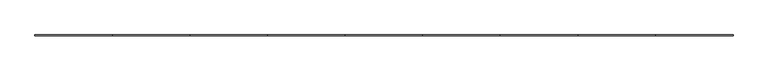
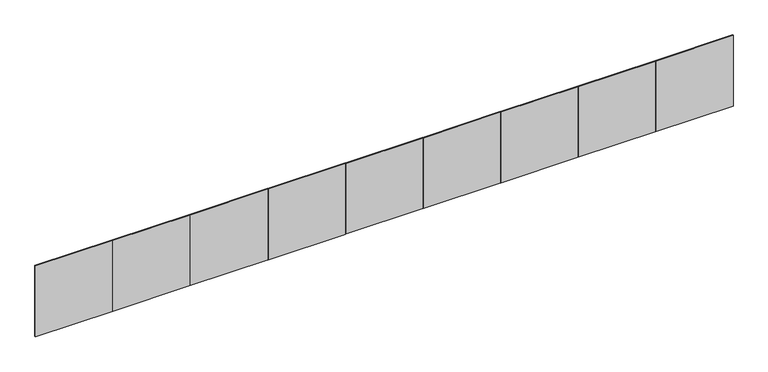
"""IFC4 building model written with IfcOpenShell, lengths in millimetres: railing geometry, ML_Painéis : ML_Painéis."""

import ifcopenshell
import ifcopenshell.guid

model = None  # the IFC model being written
_history = None  # IfcOwnerHistory: only IFC2X3 demands one
_inside = {}  # id of a spatial element -> (the spatial element, [elements in it])
_under = {}  # id of a project, library or spatial element -> (it, [spatial elements below it])
_declared = {}  # id of a project -> (the project, [libraries it declares])
_typed = {}  # id of a type object -> (the type object, [elements of that type])
_made_of = {}  # id of a material, layer set ... -> (it, [elements and type objects made of it])


def new_model(schema):
    """Start an empty IFC model of exactly this schema.

    Asked for "IFC4X3", IfcOpenShell would pick the latest addendum, in which some entities
    have other attributes; the version numbers below select the first issue.
    IFC2X3 requires an IfcOwnerHistory on every rooted entity: one is made here for all.
    """
    global model, _history
    if schema == "IFC4X3":
        model = ifcopenshell.file(schema_version=(4, 3, 0, 0))
    else:
        model = ifcopenshell.file(schema=schema)
    _inside.clear()
    _under.clear()
    _declared.clear()
    _typed.clear()
    _made_of.clear()
    _history = None
    if model.schema == "IFC2X3":
        org = make("IfcOrganization", Name="unknown")
        user = make(
            "IfcPersonAndOrganization",
            ThePerson=make("IfcPerson", FamilyName="unknown"),
            TheOrganization=org,
        )
        app = make(
            "IfcApplication",
            ApplicationDeveloper=org,
            Version="unknown",
            ApplicationFullName="unknown",
            ApplicationIdentifier="unknown",
        )
        _history = make(
            "IfcOwnerHistory",
            OwningUser=user,
            OwningApplication=app,
            ChangeAction="ADDED",
            CreationDate=0,
        )
    return model


def make(cls, **values):
    """One entity of the class cls with the attributes given. An attribute that is None is left unset."""
    return model.create_entity(
        cls, **{name: value for name, value in values.items() if value is not None}
    )


def rooted(cls, **values):
    """An entity with a GlobalId (a new one), such as an element, a storey or a relation."""
    return make(cls, GlobalId=ifcopenshell.guid.new(), OwnerHistory=_history, **values)


def si_unit(unit_type, name, prefix=None):
    """IfcSIUnit, for example si_unit("LENGTHUNIT", "METRE", prefix="MILLI")."""
    return make("IfcSIUnit", UnitType=unit_type, Prefix=prefix, Name=name)


def assignment(units):
    """IfcUnitAssignment: the units of a project."""
    return None if units is None else make("IfcUnitAssignment", Units=units)


def point(xyz):
    """IfcCartesianPoint."""
    return None if xyz is None else make("IfcCartesianPoint", Coordinates=xyz)


def direction(xyz):
    """IfcDirection."""
    return None if xyz is None else make("IfcDirection", DirectionRatios=xyz)


def frame(location, z_axis=None, x_axis=None):
    """IfcAxis2Placement3D, a coordinate frame: its origin and axes. An axis left out is left unset."""
    return make(
        "IfcAxis2Placement3D",
        Location=point(location),
        Axis=direction(z_axis),
        RefDirection=direction(x_axis),
    )


def origin():
    """The frame at (0, 0, 0) with its axes left unset."""
    return frame((0.0, 0.0, 0.0))


def place(relative_to, where):
    """IfcLocalPlacement: puts the frame where relative to a parent placement (None: the world)."""
    return make(
        "IfcLocalPlacement", PlacementRelTo=relative_to, RelativePlacement=where
    )


def context(
    kind, dimensions, precision=None, world=None, true_north=None, identifier=None
):
    """IfcGeometricRepresentationContext, for example the 3D "Model" context."""
    return make(
        "IfcGeometricRepresentationContext",
        ContextIdentifier=identifier,
        ContextType=kind,
        CoordinateSpaceDimension=dimensions,
        Precision=precision,
        WorldCoordinateSystem=world,
        TrueNorth=true_north,
    )


def project(units=None, contexts=None):
    """IfcProject with its units and contexts."""
    return rooted(
        "IfcProject",
        Name="project",
        RepresentationContexts=contexts,
        UnitsInContext=assignment(units),
    )


def spatial(cls, under=None, at=None, **own):
    """A site, building, storey or space (cls), placed at a placement, below another one or the project."""
    s = rooted(cls, ObjectPlacement=at, **own)
    if under is not None:
        _under.setdefault(under.id(), (under, []))[1].append(s)
    return s


def polyline(points):
    """IfcPolyline through the points."""
    return make("IfcPolyline", Points=[point(p) for p in points])


def outline(outer, holes=None, kind="AREA"):
    """IfcArbitraryClosedProfileDef: a profile drawn as a closed curve; with holes, ...WithVoids."""
    if holes is None:
        return make("IfcArbitraryClosedProfileDef", ProfileType=kind, OuterCurve=outer)
    return make(
        "IfcArbitraryProfileDefWithVoids",
        ProfileType=kind,
        OuterCurve=outer,
        InnerCurves=holes,
    )


def extrude(swept, where, along, depth):
    """IfcExtrudedAreaSolid: the profile swept, set in the frame where, extruded along a direction by depth."""
    return make(
        "IfcExtrudedAreaSolid",
        SweptArea=swept,
        Position=where,
        ExtrudedDirection=direction(along),
        Depth=depth,
    )


def shape(context_of_items, identifier, shape_type, items):
    """IfcShapeRepresentation: the items that make up one representation, for example the "Body"."""
    return make(
        "IfcShapeRepresentation",
        ContextOfItems=context_of_items,
        RepresentationIdentifier=identifier,
        RepresentationType=shape_type,
        Items=items,
    )


def source(mapping_origin, context_of_items, identifier, shape_type, items):
    """IfcRepresentationMap: a shape defined once, which mapped items show again and again."""
    return make(
        "IfcRepresentationMap",
        MappingOrigin=mapping_origin,
        MappedRepresentation=shape(context_of_items, identifier, shape_type, items),
    )


def transform(
    local_origin,
    x_axis=None,
    y_axis=None,
    z_axis=None,
    scale=None,
    scale2=None,
    scale3=None,
    uniform=True,
):
    """IfcCartesianTransformationOperator3D, or its non-uniform kind. x_axis, y_axis, z_axis: its Axis1, 2, 3."""
    if uniform:
        return make(
            "IfcCartesianTransformationOperator3D",
            Axis1=direction(x_axis),
            Axis2=direction(y_axis),
            LocalOrigin=point(local_origin),
            Scale=scale,
            Axis3=direction(z_axis),
        )
    return make(
        "IfcCartesianTransformationOperator3DnonUniform",
        Axis1=direction(x_axis),
        Axis2=direction(y_axis),
        LocalOrigin=point(local_origin),
        Scale=scale,
        Axis3=direction(z_axis),
        Scale2=scale2,
        Scale3=scale3,
    )


def mapped(mapping_source, mapping_target):
    """IfcMappedItem: shows the shape of a source again, moved by a transform."""
    return make(
        "IfcMappedItem", MappingSource=mapping_source, MappingTarget=mapping_target
    )


def made_of(thing, what):
    """Note that an element or type object is made of a material, layer set ...; save() writes the relation."""
    if what is not None:
        _made_of.setdefault(what.id(), (what, []))[1].append(thing)
    return thing


def element(
    cls,
    number,
    at=None,
    inside=None,
    cuts=None,
    type_object=None,
    material=None,
    context=None,
    identifier="Body",
    shape_type=None,
    held_by="IfcProductDefinitionShape",
    body=None,
    shapes=None,
    **own,
):
    """One element of the class cls, such as IfcWall. Its Tag is "e" and its number.

    at: its placement. inside: the storey or other place that contains it. cuts: it is an
    opening in that element (IfcRelVoidsElement). A single representation is given by context,
    identifier, shape_type and body (its items); several are given by shapes. held_by: the class
    of the entity that holds the representations. save() writes the other relations.
    """
    e = rooted(cls, Tag="e%d" % number, ObjectPlacement=at, **own)
    if body is not None:
        shapes = [shape(context, identifier, shape_type, body)]
    if shapes is not None:
        e.Representation = make(held_by, Representations=shapes)
    if inside is not None:
        _inside.setdefault(inside.id(), (inside, []))[1].append(e)
    if cuts is not None:
        rooted(
            "IfcRelVoidsElement", RelatingBuildingElement=cuts, RelatedOpeningElement=e
        )
    if type_object is not None:
        _typed.setdefault(type_object.id(), (type_object, []))[1].append(e)
    return made_of(e, material)


def aggregate(whole, parts):
    """IfcRelAggregates: a whole, such as a stair, and the parts it consists of."""
    return rooted("IfcRelAggregates", RelatingObject=whole, RelatedObjects=parts)


def save(model, path):
    """Write the relations noted so far, then the file.

    IfcRelAggregates (storeys below a building ...), IfcRelContainedInSpatialStructure (elements
    in a storey), IfcRelDefinesByType, IfcRelAssociatesMaterial and IfcRelDeclares: one each for
    every whole, place, type object, material and project.
    """
    for whole, parts in _under.values():
        aggregate(whole, parts)
    for where, things in _inside.values():
        rooted(
            "IfcRelContainedInSpatialStructure",
            RelatedElements=things,
            RelatingStructure=where,
        )
    for kind, things in _typed.values():
        rooted("IfcRelDefinesByType", RelatedObjects=things, RelatingType=kind)
    for what, things in _made_of.values():
        rooted("IfcRelAssociatesMaterial", RelatedObjects=things, RelatingMaterial=what)
    for by, libraries in _declared.values():
        rooted("IfcRelDeclares", RelatingContext=by, RelatedDefinitions=libraries)
    model.write(path)


def railing_be0b07b7(model_context):
    return source(origin(), model_context, "Body", "SweptSolid", [
        extrude(outline(polyline([(-4674.5702584, 2133.3602771), (-4674.5702584, 2121.3602771), (-5709.5702584, 2121.3602771), (-5709.5702584, 2133.3602771), (-4674.5702584, 2133.3602771)])), frame((0.0, 0.0, 4122.0679199), z_axis=(0.0, 0.0, 1.0), x_axis=(1.0, 0.0, 0.0)), (0.0, 0.0, 1.0), 1000.0),
        extrude(outline(polyline([(-5711.5702584, 2133.3602771), (-5711.5702584, 2121.3602771), (-6746.5702584, 2121.3602771), (-6746.5702584, 2133.3602771), (-5711.5702584, 2133.3602771)])), frame((0.0, 0.0, 4122.0679199), z_axis=(0.0, 0.0, 1.0), x_axis=(1.0, 0.0, 0.0)), (0.0, 0.0, 1.0), 1000.0),
        extrude(outline(polyline([(-6748.5702584, 2133.3602771), (-6748.5702584, 2121.3602771), (-7783.5702584, 2121.3602771), (-7783.5702584, 2133.3602771), (-6748.5702584, 2133.3602771)])), frame((0.0, 0.0, 4122.0679199), z_axis=(0.0, 0.0, 1.0), x_axis=(1.0, 0.0, 0.0)), (0.0, 0.0, 1.0), 1000.0),
        extrude(outline(polyline([(-7785.5702584, 2133.3602771), (-7785.5702584, 2121.3602771), (-8820.5702584, 2121.3602771), (-8820.5702584, 2133.3602771), (-7785.5702584, 2133.3602771)])), frame((0.0, 0.0, 4122.0679199), z_axis=(0.0, 0.0, 1.0), x_axis=(1.0, 0.0, 0.0)), (0.0, 0.0, 1.0), 1000.0),
        extrude(outline(polyline([(-8822.5702584, 2133.3602771), (-8822.5702584, 2121.3602771), (-9857.5702584, 2121.3602771), (-9857.5702584, 2133.3602771), (-8822.5702584, 2133.3602771)])), frame((0.0, 0.0, 4122.0679199), z_axis=(0.0, 0.0, 1.0), x_axis=(1.0, 0.0, 0.0)), (0.0, 0.0, 1.0), 1000.0),
        extrude(outline(polyline([(-9859.5702584, 2133.3602771), (-9859.5702584, 2121.3602771), (-10894.5702584, 2121.3602771), (-10894.5702584, 2133.3602771), (-9859.5702584, 2133.3602771)])), frame((0.0, 0.0, 4122.0679199), z_axis=(0.0, 0.0, 1.0), x_axis=(1.0, 0.0, 0.0)), (0.0, 0.0, 1.0), 1000.0),
        extrude(outline(polyline([(-10896.5702584, 2133.3602771), (-10896.5702584, 2121.3602771), (-11931.5702584, 2121.3602771), (-11931.5702584, 2133.3602771), (-10896.5702584, 2133.3602771)])), frame((0.0, 0.0, 4122.0679199), z_axis=(0.0, 0.0, 1.0), x_axis=(1.0, 0.0, 0.0)), (0.0, 0.0, 1.0), 1000.0),
        extrude(outline(polyline([(-11933.5702584, 2133.3602771), (-11933.5702584, 2121.3602771), (-12968.5702584, 2121.3602771), (-12968.5702584, 2133.3602771), (-11933.5702584, 2133.3602771)])), frame((0.0, 0.0, 4122.0679199), z_axis=(0.0, 0.0, 1.0), x_axis=(1.0, 0.0, 0.0)), (0.0, 0.0, 1.0), 1000.0),
        extrude(outline(polyline([(-12970.5702584, 2133.3602771), (-12970.5702584, 2121.3602771), (-14005.5702584, 2121.3602771), (-14005.5702584, 2133.3602771), (-12970.5702584, 2133.3602771)])), frame((0.0, 0.0, 4122.0679199), z_axis=(0.0, 0.0, 1.0), x_axis=(1.0, 0.0, 0.0)), (0.0, 0.0, 1.0), 1000.0),
    ])


if __name__ == "__main__":
    model = new_model("IFC4")
    model_context = context("Model", 3, world=origin())
    ifc_project = project(units=[si_unit("LENGTHUNIT", "METRE", prefix="MILLI")], contexts=[model_context])
    site = spatial("IfcSite", under=ifc_project)
    building = spatial("IfcBuilding", under=site)
    placement = place(None, origin())
    railing_shape = railing_be0b07b7(model_context)
    element("IfcRailing", 1, ObjectType="ML_Painéis : ML_Painéis", at=placement, inside=building, context=model_context, shape_type="MappedRepresentation", body=[
        mapped(railing_shape, transform((0.0, 0.0, 0.0), x_axis=(1.0, 0.0, 0.0), y_axis=(0.0, 1.0, 0.0), z_axis=(0.0, 0.0, 1.0))),
    ])
    save(model, "model.ifc")

# Revit data of these elements
# Type "ML_Painéis : ML_Painéis"
#   ME_Área [instance default] = 9.315 m²
#   ME_Espessura [instance default] = 0.012 m
#   ME_Dist Painéis [instance default] = 0.002 m
#   ME_Compr Painéis [instance default] = 1.035 m
#   ME_Compr [instance default] = 9.335 m
#   ME_Altura [instance default] = 1.00 m
#   ME_Quant Painéis [instance default] = 9
#   ME_Painel Único [instance default] = no
#   ME_Paineis Vários [instance default] = yes
#   ME_Material Tipo Vidro [instance default] = .VIDRO GENÉRICO
# Element 1 (IfcRailing, "ML_Painéis : ML_Painéis")
#   Materials on its faces: ".VIDRO GENÉRICO"
# Materials
#   ".VIDRO GENÉRICO": class ".CC_VIDRO", colour RGB 0 128 192, transparency 0.9, Description = "Vidro comum", Cost = 0
